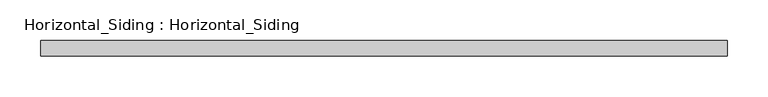
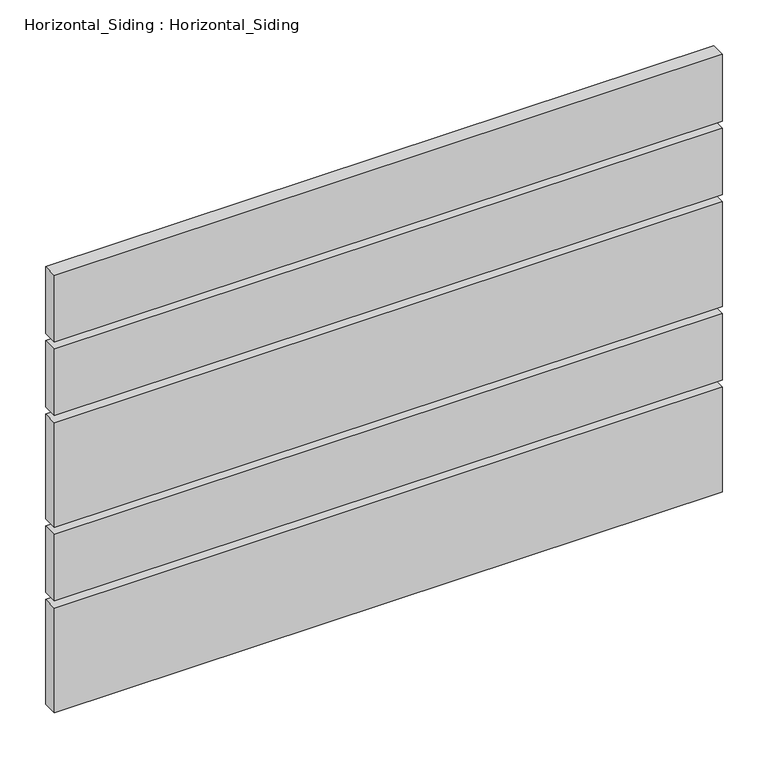
"""IFC4 building model written with IfcOpenShell, lengths in millimetres: plate geometry, Horizontal_Siding : Horizontal_Siding."""

from ifc_helpers import new_model, si_unit, frame, origin, place, context, project, spatial, polyline, outline, extrude, source, transform, mapped, element, save


def horizontal_siding_horizontal_siding_d6c4737b(model_context):
    return source(origin(), model_context, "Body", "SweptSolid", [
        extrude(outline(polyline([(421.48125, -19.05), (-421.48125, -19.05), (-421.48125, 0.0), (421.48125, 0.0), (421.48125, -19.05)])), frame((0.0, 0.0, 9.525), z_axis=(0.0, 0.0, 1.0), x_axis=(1.0, 0.0, 0.0)), (0.0, 0.0, 1.0), 139.7),
        extrude(outline(polyline([(421.48125, -19.05), (-421.48125, -19.05), (-421.48125, 0.0), (421.48125, 0.0), (421.48125, -19.05)])), frame((0.0, 0.0, 158.75), z_axis=(0.0, 0.0, 1.0), x_axis=(1.0, 0.0, 0.0)), (0.0, 0.0, 1.0), 88.9),
        extrude(outline(polyline([(421.48125, -19.05), (-421.48125, -19.05), (-421.48125, 0.0), (421.48125, 0.0), (421.48125, -19.05)])), frame((0.0, 0.0, 257.175), z_axis=(0.0, 0.0, 1.0), x_axis=(1.0, 0.0, 0.0)), (0.0, 0.0, 1.0), 139.7),
        extrude(outline(polyline([(421.48125, -19.05), (-421.48125, -19.05), (-421.48125, 0.0), (421.48125, 0.0), (421.48125, -19.05)])), frame((0.0, 0.0, 406.4), z_axis=(0.0, 0.0, 1.0), x_axis=(1.0, 0.0, 0.0)), (0.0, 0.0, 1.0), 88.9),
        extrude(outline(polyline([(421.48125, -19.05), (-421.48125, -19.05), (-421.48125, 0.0), (421.48125, 0.0), (421.48125, -19.05)])), frame((0.0, 0.0, 504.825), z_axis=(0.0, 0.0, 1.0), x_axis=(1.0, 0.0, 0.0)), (0.0, 0.0, 1.0), 88.9),
    ])


if __name__ == "__main__":
    model = new_model("IFC4")
    model_context = context("Model", 3, world=origin())
    ifc_project = project(units=[si_unit("LENGTHUNIT", "METRE", prefix="MILLI")], contexts=[model_context])
    site = spatial("IfcSite", under=ifc_project)
    building = spatial("IfcBuilding", under=site)
    placement = place(None, origin())
    horizontal_siding_horizontal_siding_shape = horizontal_siding_horizontal_siding_d6c4737b(model_context)
    element("IfcPlate", 1, ObjectType="Horizontal_Siding : Horizontal_Siding", at=placement, inside=building, context=model_context, shape_type="MappedRepresentation", body=[
        mapped(horizontal_siding_horizontal_siding_shape, transform((0.0, 0.0, 0.0), x_axis=(1.0, 0.0, 0.0), y_axis=(0.0, 1.0, 0.0), z_axis=(0.0, 0.0, 1.0))),
    ])
    save(model, "model.ifc")

# Revit data of these elements
# Type "Horizontal_Siding : Horizontal_Siding"
#   Analytic Construction = "<None>"
#   extend = 0' - 2 3/4"
#   Width_2 = 0' - 3 1/2"
#   Width_1 = 0' - 5 1/2"
#   Gap = 0' - 0 3/8"
#   Plank Material = SLOTTED WOOD FENCE (THERMALLY MODIFIED WOOD: ARBOR WOOD)\n(EXTERIOR STAIN : PENOFIN VERDE EXT. STAIN - COLOR: CEDAR)
# Element 1 (IfcPlate, "Horizontal_Siding : Horizontal_Siding")
#   Materials on its faces: "SLOTTED WOOD FENCE (THERMALLY MODIFIED WOOD: ARBOR WOOD)\n(EXTERIOR STAIN : PENOFIN VERDE EXT. STAIN - COLOR: CEDAR)"
# Materials
#   "SLOTTED WOOD FENCE (THERMALLY MODIFIED WOOD: ARBOR WOOD)\n(EXTERIOR STAIN : PENOFIN VERDE EXT. STAIN - COLOR: CEDAR)": class "Wood", colour RGB 164 134 123, transparency 0, Description = "Pinus Echinata", Cost = 0
